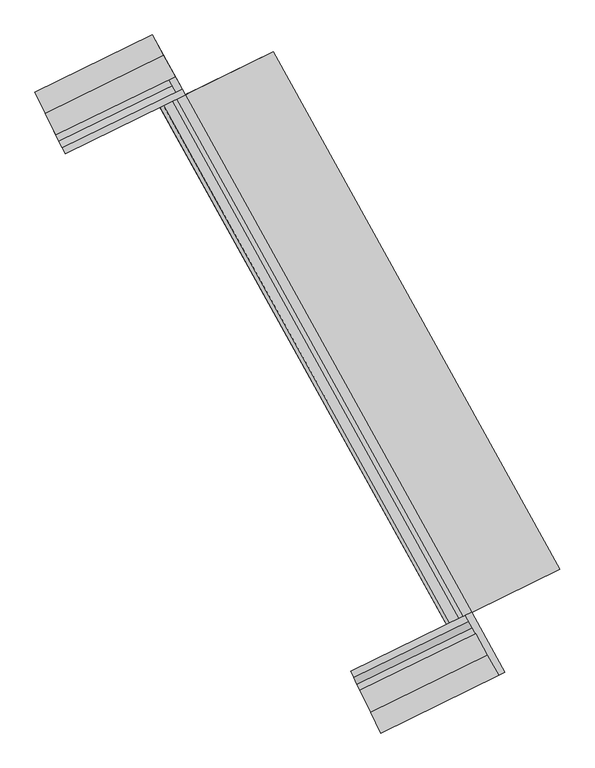
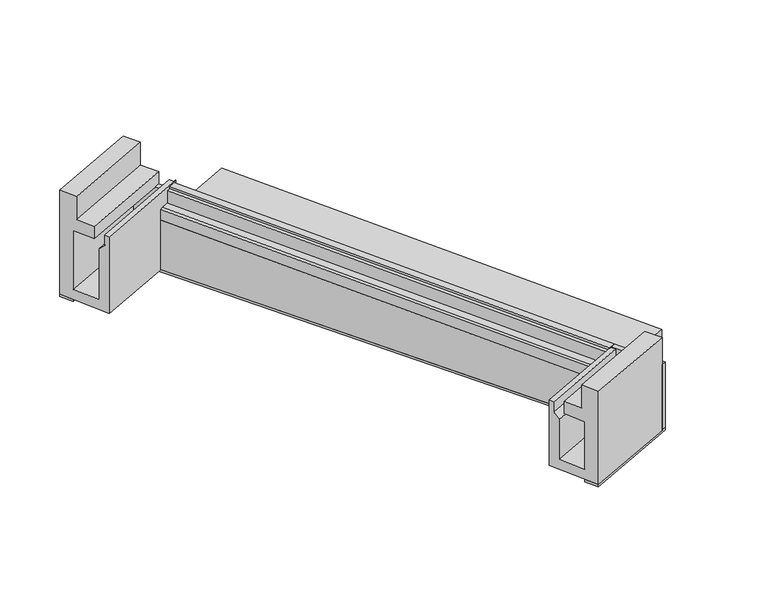
"""IFC4 building model written with IfcOpenShell, lengths in millimetres: beam geometry, KNA_SF-LH-as1 : KNA_SF-LH-as1."""

from ifc_helpers import new_model, si_unit, frame, origin, place, context, project, spatial, polyline, outline, extrude, faceted_brep, source, transform, mapped, element, save


def beam_d1400e5c(model_context):
    return source(origin(), model_context, "Body", "SolidModel", [
        extrude(outline(polyline([(121503.0616469, -57693.8883639), (120790.1519014, -56406.1454116), (120921.3836354, -56333.4939699), (121634.2933809, -57621.2369222), (121503.0616469, -57693.8883639)])), frame((0.0, 0.0, 2350.0), z_axis=(0.0, 0.0, 1.0), x_axis=(1.0, 0.0, 0.0)), (0.0, 0.0, 1.0), 1980.3403564),
        faceted_brep([(121260.5753389, -57255.880557, 5155.0), (118751.9287504, -58482.1096271, 5155.0), (118971.5019672, -58931.3173769, 5155.0), (121503.0616469, -57693.8883639, 5155.0), (121260.5753389, -57255.880557, 4471.289564), (118751.9287504, -58482.1096271, 4471.289564), (121007.4627589, -56798.6783052, 4458.9535606), (118522.7333626, -58013.2166269, 4458.9535606), (121007.4627589, -56798.6783052, 4088.9535606), (118522.7333626, -58013.2166269, 4088.9535606), (121309.0726005, -57343.4821184, 4088.9535606), (118795.8433937, -58571.9511771, 4088.9535606), (121309.0726005, -57343.4821184, 2650.0), (118795.8433937, -58571.9511771, 2650.0), (120934.7168665, -56667.2759631, 2650.0), (118456.8613975, -57878.4543019, 2650.0), (120934.7168665, -56667.2759631, 3852.4579638), (118456.8613975, -57878.4543019, 3852.4579638), (120856.6803591, -56526.3170786, 4013.3670645), (118386.1987398, -57733.8910719, 4013.3670645), (120856.6803591, -56526.3170786, 4327.6885528), (118386.1987398, -57733.8910719, 4327.6885528), (120789.2250817, -56404.471279, 4324.4009701), (118325.1174674, -57608.9296521, 4324.4009701), (120789.2250817, -56404.471279, 2350.0), (118325.1174674, -57608.9296521, 2350.0), (121503.0616469, -57693.8883639, 2350.0), (118971.5019672, -58931.3173769, 2350.0)], [[[0, 1, 2, 3]], [[1, 0, 4, 5]], [[5, 4, 6, 7]], [[7, 6, 8, 9]], [[9, 8, 10, 11]], [[11, 10, 12, 13]], [[13, 12, 14, 15]], [[15, 14, 16, 17]], [[17, 16, 18, 19]], [[19, 18, 20, 21]], [[21, 20, 22, 23]], [[23, 22, 24, 25]], [[25, 24, 26, 27]], [[27, 26, 3, 2]], [[0, 3, 26, 24, 22, 20, 18, 16, 14, 12, 10, 8, 6, 4]], [[2, 1, 5, 7, 9, 11, 13, 15, 17, 19, 21, 23, 25, 27]]]),
        extrude(outline(polyline([(114120.8084861, -44359.1786908), (114255.746009, -44293.2210888), (114775.5935278, -45232.2319282), (114640.6560048, -45298.1895302), (114120.8084861, -44359.1786908)])), frame((0.0, 0.0, 2650.0), z_axis=(0.0, 0.0, 1.0), x_axis=(1.0, 0.0, 0.0)), (0.0, 0.0, 1.0), 1773.9535606),
        faceted_brep([(114831.5585968, -45204.8761441, 4659.4009701), (114831.5585968, -45204.8761441, 2350.0), (114829.321813, -45200.3000824, 2350.0), (114829.321813, -45200.3000824, 4659.5213607), (114061.7569626, -43942.8148433, 5490.0), (111546.1935639, -45172.4248575, 5490.0), (111765.7667807, -45621.6326073, 5490.0), (114304.2432706, -44380.8226502, 5490.0), (111765.7667807, -45621.6326073, 4806.289564), (114304.2432706, -44380.8226502, 4806.289564), (111994.9621685, -46090.5256075, 4793.9535606), (114557.3558506, -44838.024902, 4793.9535606), (111994.9621685, -46090.5256075, 4423.9535606), (114557.3558506, -44838.024902, 4423.9535606), (111721.8521373, -45531.7910573, 4423.9535606), (114255.746009, -44293.2210888, 4423.9535606), (111721.8521373, -45531.7910573, 2650.0), (114255.746009, -44293.2210888, 2650.0), (112060.8341335, -46225.2879325, 2650.0), (114630.101743, -44969.4272441, 2650.0), (112060.8341335, -46225.2879325, 4187.4579638), (114630.101743, -44969.4272441, 4187.4579638), (112131.4967912, -46369.8511625, 4348.3670645), (114708.1382505, -45110.3861286, 4348.3670645), (112131.4967912, -46369.8511625, 4662.6885528), (114708.1382505, -45110.3861286, 4662.6885528), (114774.6667081, -45230.5577956, 4659.4461407), (112192.5780636, -46494.8125823, 4659.4009701), (112192.5780636, -46494.8125823, 2350.0), (111546.1935639, -45172.4248575, 2350.0), (114061.7569626, -43942.8148433, 2350.0), (114774.6667081, -45230.5577956, 2350.0)], [[[0, 1, 2, 3]], [[4, 5, 6, 7]], [[7, 6, 8, 9]], [[9, 8, 10, 11]], [[11, 10, 12, 13]], [[13, 12, 14, 15]], [[15, 14, 16, 17]], [[17, 16, 18, 19]], [[19, 18, 20, 21]], [[21, 20, 22, 23]], [[23, 22, 24, 25]], [[0, 3, 26, 25, 24, 27]], [[1, 0, 27, 28]], [[2, 1, 28, 29, 30, 31]], [[5, 4, 30, 29]], [[26, 31, 30, 4, 7, 9, 11, 13, 15, 17, 19, 21, 23, 25]], [[31, 26, 3, 2]], [[6, 5, 29, 28, 27, 24, 22, 20, 18, 16, 14, 12, 10, 8]]]),
        faceted_brep([(120385.3393325, -56604.0182177, 3551.6043595), (114234.9166164, -45494.3882036, 3848.8430242), (114234.9166164, -45494.3882036, 2350.0), (120385.3393325, -56604.0182177, 2350.0), (122814.2147455, -55416.7813814, 3548.3806676), (116663.7920294, -44307.1513674, 3845.6193324), (122814.2147455, -55416.7813814, 2350.0), (116663.7920294, -44307.1513674, 2350.0)], [[[0, 1, 2, 3]], [[1, 0, 4, 5]], [[5, 4, 6, 7]], [[3, 2, 7, 6]], [[2, 1, 5, 7]], [[0, 3, 6, 4]]]),
        faceted_brep([(120925.0894243, -56340.1878096, 3550.8879835), (114774.6667081, -45230.5577956, 3848.1266482), (114774.6667081, -45230.5577956, 4627.3400287), (120925.0894243, -56340.1878096, 4330.101364), (114594.7500109, -45318.5012649, 4627.5788207), (120745.1727271, -56428.131279, 4330.340156), (114594.7500109, -45318.5012649, 4557.5596466), (120745.1727271, -56428.131279, 4260.3209819), (114504.7916623, -45362.4729996, 4557.6790426), (120655.2143784, -56472.1030137, 4260.4403779), (114504.7916623, -45362.4729996, 4187.5776937), (120655.2143784, -56472.1030137, 3890.339029), (114306.8832953, -45459.2108159, 4187.8403649), (120457.3060114, -56568.84083, 3890.6017002), (114234.9166164, -45494.3882036, 4162.9290338), (120385.3393325, -56604.0182177, 3865.6903691), (114234.9166164, -45494.3882036, 3848.8430242), (120385.3393325, -56604.0182177, 3551.6043595)], [[[0, 1, 2, 3]], [[3, 2, 4, 5]], [[5, 4, 6, 7]], [[7, 6, 8, 9]], [[9, 8, 10, 11]], [[11, 10, 12, 13]], [[13, 12, 14, 15]], [[15, 14, 16, 17]], [[1, 0, 17, 16]], [[2, 1, 16, 14, 12, 10, 8, 6, 4]], [[0, 3, 5, 7, 9, 11, 13, 15, 17]]]),
        extrude(outline(polyline([(122814.2147455, -55416.7813814), (120925.0894243, -56340.1878096), (121637.9991698, -57627.9307619), (118971.5019672, -58931.3173769), (118795.8433937, -58571.9511771), (120904.2600317, -57541.3549244), (113715.9959172, -44557.0514969), (111721.8521373, -45531.7910573), (111546.1935639, -45172.4248575), (114061.7569626, -43942.8148433), (114774.6667081, -45230.5577956), (116663.7920294, -44307.1513674), (122814.2147455, -55416.7813814)])), frame((0.0, 0.0, 2280.0), z_axis=(0.0, 0.0, 1.0), x_axis=(1.0, 0.0, 0.0)), (0.0, 0.0, 1.0), 70.0),
    ])


if __name__ == "__main__":
    model = new_model("IFC4")
    model_context = context("Model", 3, world=origin())
    ifc_project = project(units=[si_unit("LENGTHUNIT", "METRE", prefix="MILLI")], contexts=[model_context])
    site = spatial("IfcSite", under=ifc_project)
    building = spatial("IfcBuilding", under=site)
    placement = place(None, origin())
    beam_shape = beam_d1400e5c(model_context)
    element("IfcBeam", 1, ObjectType="KNA_SF-LH-as1 : KNA_SF-LH-as1", at=placement, inside=building, context=model_context, shape_type="MappedRepresentation", body=[
        mapped(beam_shape, transform((0.0, 0.0, 0.0), x_axis=(1.0, 0.0, 0.0), y_axis=(0.0, 1.0, 0.0), z_axis=(0.0, 0.0, 1.0))),
    ])
    save(model, "model.ifc")

# Revit data of these elements
# Element 1 (IfcBeam, "KNA_SF-LH-as1 : KNA_SF-LH-as1")
#   Materials on its faces: "Beton_Bestaande Constructie", "Beton_In-Situ_Werkvloer"
# Materials
#   "Beton_Bestaande Constructie": class "Concrete", colour RGB 102 102 102, transparency 0, Description = "Beton", Cost = 0
#   "Beton_In-Situ_Werkvloer": class "Concrete", colour RGB 128 128 128, transparency 0, Description = "Beton", Cost = 0
